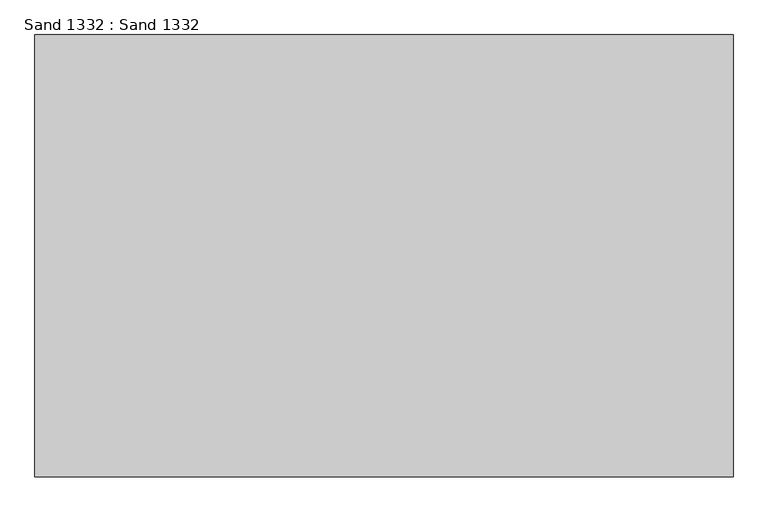
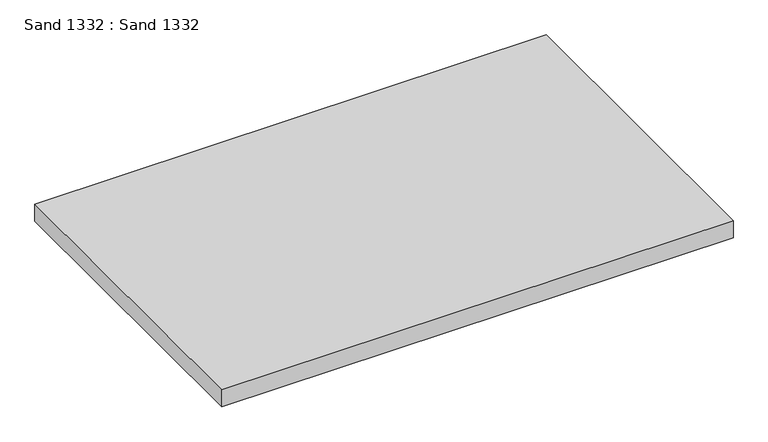
"""IFC4 building model written with IfcOpenShell, lengths in millimetres: proxy geometry, Sand 1332 : Sand 1332."""

from ifc_helpers import new_model, si_unit, frame, origin, place, context, project, spatial, polyline, outline, extrude, source, transform, mapped, element, save


def sand_1332_sand_1332_1bed2853(model_context):
    return source(origin(), model_context, "Body", "SweptSolid", [
        extrude(outline(polyline([(3694.2883192, 9730.3375834), (3694.2883192, 10997.0939628), (5694.2883192, 10997.0939628), (5694.2883192, 9730.3375834), (3694.2883192, 9730.3375834)])), frame((0.0, 0.0, 36105.4523605), z_axis=(0.0, 0.0, 1.0), x_axis=(1.0, 0.0, 0.0)), (0.0, 0.0, 1.0), 70.2358801),
    ])


if __name__ == "__main__":
    model = new_model("IFC4")
    model_context = context("Model", 3, world=origin())
    ifc_project = project(units=[si_unit("LENGTHUNIT", "METRE", prefix="MILLI")], contexts=[model_context])
    site = spatial("IfcSite", under=ifc_project)
    building = spatial("IfcBuilding", under=site)
    placement = place(None, origin())
    sand_1332_sand_1332_shape = sand_1332_sand_1332_1bed2853(model_context)
    element("IfcBuildingElementProxy", 1, Name="Sand 1332 : Sand 1332", ObjectType="Sand 1332 : Sand 1332", at=placement, inside=building, context=model_context, shape_type="MappedRepresentation", body=[
        mapped(sand_1332_sand_1332_shape, transform((0.0, 0.0, 0.0), x_axis=(1.0, 0.0, 0.0), y_axis=(0.0, 1.0, 0.0), z_axis=(0.0, 0.0, 1.0))),
    ])
    save(model, "model.ifc")

# Revit data of these elements
# Type "Sand 1332 : Sand 1332"
#   NameOverride = "Sand"
# Element 1 (IfcBuildingElementProxy, "Sand 1332 : Sand 1332")
#   Materials on its faces: "2\" SAND LAYER"
# Materials
#   "2\" SAND LAYER": class "Unassigned", colour RGB 239 206 153, transparency 0, Cost = 0
